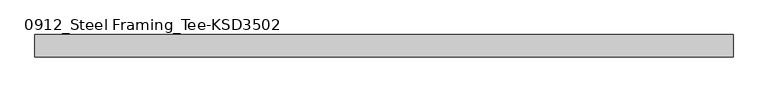
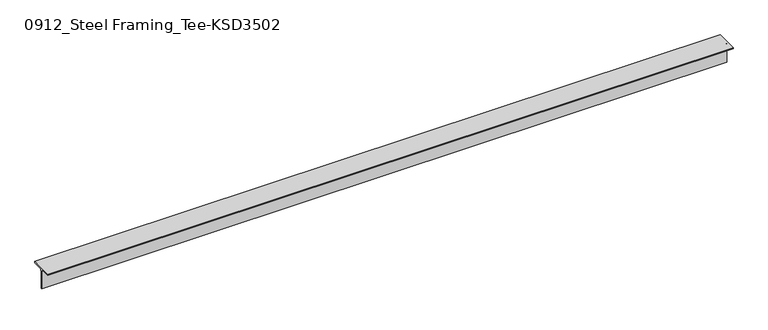
"""IFC4 building model written with IfcOpenShell, lengths in millimetres: member geometry, 0912_Steel Framing_Tee-KSD3502 : H_SB_ASB_CT-150x150x6.5x9."""

import ifcopenshell
import ifcopenshell.guid

model = None  # the IFC model being written
_history = None  # IfcOwnerHistory: only IFC2X3 demands one
_inside = {}  # id of a spatial element -> (the spatial element, [elements in it])
_under = {}  # id of a project, library or spatial element -> (it, [spatial elements below it])
_declared = {}  # id of a project -> (the project, [libraries it declares])
_typed = {}  # id of a type object -> (the type object, [elements of that type])
_made_of = {}  # id of a material, layer set ... -> (it, [elements and type objects made of it])


def new_model(schema):
    """Start an empty IFC model of exactly this schema.

    Asked for "IFC4X3", IfcOpenShell would pick the latest addendum, in which some entities
    have other attributes; the version numbers below select the first issue.
    IFC2X3 requires an IfcOwnerHistory on every rooted entity: one is made here for all.
    """
    global model, _history
    if schema == "IFC4X3":
        model = ifcopenshell.file(schema_version=(4, 3, 0, 0))
    else:
        model = ifcopenshell.file(schema=schema)
    _inside.clear()
    _under.clear()
    _declared.clear()
    _typed.clear()
    _made_of.clear()
    _history = None
    if model.schema == "IFC2X3":
        org = make("IfcOrganization", Name="unknown")
        user = make(
            "IfcPersonAndOrganization",
            ThePerson=make("IfcPerson", FamilyName="unknown"),
            TheOrganization=org,
        )
        app = make(
            "IfcApplication",
            ApplicationDeveloper=org,
            Version="unknown",
            ApplicationFullName="unknown",
            ApplicationIdentifier="unknown",
        )
        _history = make(
            "IfcOwnerHistory",
            OwningUser=user,
            OwningApplication=app,
            ChangeAction="ADDED",
            CreationDate=0,
        )
    return model


def make(cls, **values):
    """One entity of the class cls with the attributes given. An attribute that is None is left unset."""
    return model.create_entity(
        cls, **{name: value for name, value in values.items() if value is not None}
    )


def rooted(cls, **values):
    """An entity with a GlobalId (a new one), such as an element, a storey or a relation."""
    return make(cls, GlobalId=ifcopenshell.guid.new(), OwnerHistory=_history, **values)


def si_unit(unit_type, name, prefix=None):
    """IfcSIUnit, for example si_unit("LENGTHUNIT", "METRE", prefix="MILLI")."""
    return make("IfcSIUnit", UnitType=unit_type, Prefix=prefix, Name=name)


def assignment(units):
    """IfcUnitAssignment: the units of a project."""
    return None if units is None else make("IfcUnitAssignment", Units=units)


def point(xyz):
    """IfcCartesianPoint."""
    return None if xyz is None else make("IfcCartesianPoint", Coordinates=xyz)


def direction(xyz):
    """IfcDirection."""
    return None if xyz is None else make("IfcDirection", DirectionRatios=xyz)


def frame(location, z_axis=None, x_axis=None):
    """IfcAxis2Placement3D, a coordinate frame: its origin and axes. An axis left out is left unset."""
    return make(
        "IfcAxis2Placement3D",
        Location=point(location),
        Axis=direction(z_axis),
        RefDirection=direction(x_axis),
    )


def frame_2d(location, x_axis=None):
    """IfcAxis2Placement2D, a coordinate frame in the plane: its origin and x axis."""
    return make(
        "IfcAxis2Placement2D", Location=point(location), RefDirection=direction(x_axis)
    )


def origin():
    """The frame at (0, 0, 0) with its axes left unset."""
    return frame((0.0, 0.0, 0.0))


def place(relative_to, where):
    """IfcLocalPlacement: puts the frame where relative to a parent placement (None: the world)."""
    return make(
        "IfcLocalPlacement", PlacementRelTo=relative_to, RelativePlacement=where
    )


def context(
    kind, dimensions, precision=None, world=None, true_north=None, identifier=None
):
    """IfcGeometricRepresentationContext, for example the 3D "Model" context."""
    return make(
        "IfcGeometricRepresentationContext",
        ContextIdentifier=identifier,
        ContextType=kind,
        CoordinateSpaceDimension=dimensions,
        Precision=precision,
        WorldCoordinateSystem=world,
        TrueNorth=true_north,
    )


def project(units=None, contexts=None):
    """IfcProject with its units and contexts."""
    return rooted(
        "IfcProject",
        Name="project",
        RepresentationContexts=contexts,
        UnitsInContext=assignment(units),
    )


def spatial(cls, under=None, at=None, **own):
    """A site, building, storey or space (cls), placed at a placement, below another one or the project."""
    s = rooted(cls, ObjectPlacement=at, **own)
    if under is not None:
        _under.setdefault(under.id(), (under, []))[1].append(s)
    return s


def polyline(points):
    """IfcPolyline through the points."""
    return make("IfcPolyline", Points=[point(p) for p in points])


def circle_curve(where, radius):
    """IfcCircle in the frame where."""
    return make("IfcCircle", Position=where, Radius=radius)


def trimmed(basis, trim1, trim2, sense, master):
    """IfcTrimmedCurve: the piece of a basis curve between two trims."""
    return make(
        "IfcTrimmedCurve",
        BasisCurve=basis,
        Trim1=trim1,
        Trim2=trim2,
        SenseAgreement=sense,
        MasterRepresentation=master,
    )


def segment(curve, same_sense, transition):
    """IfcCompositeCurveSegment."""
    return make(
        "IfcCompositeCurveSegment",
        Transition=transition,
        SameSense=same_sense,
        ParentCurve=curve,
    )


def composite_curve(segments, self_intersect=None):
    """IfcCompositeCurve: segments joined end to end."""
    return make("IfcCompositeCurve", Segments=segments, SelfIntersect=self_intersect)


def outline(outer, holes=None, kind="AREA"):
    """IfcArbitraryClosedProfileDef: a profile drawn as a closed curve; with holes, ...WithVoids."""
    if holes is None:
        return make("IfcArbitraryClosedProfileDef", ProfileType=kind, OuterCurve=outer)
    return make(
        "IfcArbitraryProfileDefWithVoids",
        ProfileType=kind,
        OuterCurve=outer,
        InnerCurves=holes,
    )


def extrude(swept, where, along, depth):
    """IfcExtrudedAreaSolid: the profile swept, set in the frame where, extruded along a direction by depth."""
    return make(
        "IfcExtrudedAreaSolid",
        SweptArea=swept,
        Position=where,
        ExtrudedDirection=direction(along),
        Depth=depth,
    )


def shape(context_of_items, identifier, shape_type, items):
    """IfcShapeRepresentation: the items that make up one representation, for example the "Body"."""
    return make(
        "IfcShapeRepresentation",
        ContextOfItems=context_of_items,
        RepresentationIdentifier=identifier,
        RepresentationType=shape_type,
        Items=items,
    )


def source(mapping_origin, context_of_items, identifier, shape_type, items):
    """IfcRepresentationMap: a shape defined once, which mapped items show again and again."""
    return make(
        "IfcRepresentationMap",
        MappingOrigin=mapping_origin,
        MappedRepresentation=shape(context_of_items, identifier, shape_type, items),
    )


def transform(
    local_origin,
    x_axis=None,
    y_axis=None,
    z_axis=None,
    scale=None,
    scale2=None,
    scale3=None,
    uniform=True,
):
    """IfcCartesianTransformationOperator3D, or its non-uniform kind. x_axis, y_axis, z_axis: its Axis1, 2, 3."""
    if uniform:
        return make(
            "IfcCartesianTransformationOperator3D",
            Axis1=direction(x_axis),
            Axis2=direction(y_axis),
            LocalOrigin=point(local_origin),
            Scale=scale,
            Axis3=direction(z_axis),
        )
    return make(
        "IfcCartesianTransformationOperator3DnonUniform",
        Axis1=direction(x_axis),
        Axis2=direction(y_axis),
        LocalOrigin=point(local_origin),
        Scale=scale,
        Axis3=direction(z_axis),
        Scale2=scale2,
        Scale3=scale3,
    )


def mapped(mapping_source, mapping_target):
    """IfcMappedItem: shows the shape of a source again, moved by a transform."""
    return make(
        "IfcMappedItem", MappingSource=mapping_source, MappingTarget=mapping_target
    )


def made_of(thing, what):
    """Note that an element or type object is made of a material, layer set ...; save() writes the relation."""
    if what is not None:
        _made_of.setdefault(what.id(), (what, []))[1].append(thing)
    return thing


def element(
    cls,
    number,
    at=None,
    inside=None,
    cuts=None,
    type_object=None,
    material=None,
    context=None,
    identifier="Body",
    shape_type=None,
    held_by="IfcProductDefinitionShape",
    body=None,
    shapes=None,
    **own,
):
    """One element of the class cls, such as IfcWall. Its Tag is "e" and its number.

    at: its placement. inside: the storey or other place that contains it. cuts: it is an
    opening in that element (IfcRelVoidsElement). A single representation is given by context,
    identifier, shape_type and body (its items); several are given by shapes. held_by: the class
    of the entity that holds the representations. save() writes the other relations.
    """
    e = rooted(cls, Tag="e%d" % number, ObjectPlacement=at, **own)
    if body is not None:
        shapes = [shape(context, identifier, shape_type, body)]
    if shapes is not None:
        e.Representation = make(held_by, Representations=shapes)
    if inside is not None:
        _inside.setdefault(inside.id(), (inside, []))[1].append(e)
    if cuts is not None:
        rooted(
            "IfcRelVoidsElement", RelatingBuildingElement=cuts, RelatedOpeningElement=e
        )
    if type_object is not None:
        _typed.setdefault(type_object.id(), (type_object, []))[1].append(e)
    return made_of(e, material)


def aggregate(whole, parts):
    """IfcRelAggregates: a whole, such as a stair, and the parts it consists of."""
    return rooted("IfcRelAggregates", RelatingObject=whole, RelatedObjects=parts)


def save(model, path):
    """Write the relations noted so far, then the file.

    IfcRelAggregates (storeys below a building ...), IfcRelContainedInSpatialStructure (elements
    in a storey), IfcRelDefinesByType, IfcRelAssociatesMaterial and IfcRelDeclares: one each for
    every whole, place, type object, material and project.
    """
    for whole, parts in _under.values():
        aggregate(whole, parts)
    for where, things in _inside.values():
        rooted(
            "IfcRelContainedInSpatialStructure",
            RelatedElements=things,
            RelatingStructure=where,
        )
    for kind, things in _typed.values():
        rooted("IfcRelDefinesByType", RelatedObjects=things, RelatingType=kind)
    for what, things in _made_of.values():
        rooted("IfcRelAssociatesMaterial", RelatedObjects=things, RelatingMaterial=what)
    for by, libraries in _declared.values():
        rooted("IfcRelDeclares", RelatingContext=by, RelatedDefinitions=libraries)
    model.write(path)


def member_0912_steel_framing_tee_ksd3502_358c1067(model_context):
    return source(origin(), model_context, "Body", "SweptSolid", [
        extrude(outline(composite_curve([segment(polyline([(-75.0, 75.0), (75.0, 75.0), (75.0, 66.0), (16.25, 66.0)]), True, "CONTINUOUS"), segment(trimmed(circle_curve(frame_2d((16.25, 53.0)), 13.0), [point((16.25, 66.0))], [point((3.25, 53.0))], True, "CARTESIAN"), True, "CONTINUOUS"), segment(polyline([(3.25, 53.0), (3.25, -75.0), (-3.25, -75.0), (-3.25, 53.0)]), True, "CONTINUOUS"), segment(trimmed(circle_curve(frame_2d((-16.25, 53.0)), 13.0), [point((-3.25, 53.0))], [point((-16.25, 66.0))], True, "CARTESIAN"), True, "CONTINUOUS"), segment(polyline([(-16.25, 66.0), (-75.0, 66.0), (-75.0, 75.0)]), True, "CONTINUOUS")], self_intersect=False)), frame((-2342.2, 0.0, 0.0), z_axis=(1.0, 0.0, 0.0), x_axis=(0.0, 1.0, 0.0)), (0.0, 0.0, 1.0), 4645.3),
    ])


if __name__ == "__main__":
    model = new_model("IFC4")
    model_context = context("Model", 3, world=origin())
    ifc_project = project(units=[si_unit("LENGTHUNIT", "METRE", prefix="MILLI")], contexts=[model_context])
    site = spatial("IfcSite", under=ifc_project)
    building = spatial("IfcBuilding", under=site)
    placement = place(None, origin())
    member_0912_steel_framing_tee_ksd3502_shape = member_0912_steel_framing_tee_ksd3502_358c1067(model_context)
    element("IfcMember", 1, ObjectType="0912_Steel Framing_Tee-KSD3502 : H_SB_ASB_CT-150x150x6.5x9", at=placement, inside=building, context=model_context, shape_type="MappedRepresentation", body=[
        mapped(member_0912_steel_framing_tee_ksd3502_shape, transform((0.0, 0.0, 0.0), x_axis=(1.0, 0.0, 0.0), y_axis=(0.0, 1.0, 0.0), z_axis=(0.0, 0.0, 1.0))),
    ])
    save(model, "model.ifc")

# Revit data of these elements
# Type "0912_Steel Framing_Tee-KSD3502 : H_SB_ASB_CT-150x150x6.5x9"
#   H_WM Code_1 = "S01AA003-00001 | Main Steel Structure Fabrication Work | Shelter/Building | Light Steel - Standard (30KG/M>Weight) | Material: (   )"
#   H_WM Code_2 = "S03AA029-00001 | Main Steel Structure Erection Work | Shelter/Building | Light Steel (30KG/M>Weight) | Material: (   )"
#   H_WM Code_3 = "S01AA010-00001 | Main Steel Structure Fabrication Work | Shelter/Building | Steel Painting/Coating | for Non-Fireproofed Steel Surface, Surface Preparation, Primer, Second & Final Coat | Material: (   )"
#   H_Q'ty Cal Type Tag = "SB-Q2"
#   Width = 15.0 cm
#   Web Thickness = 0.65 cm
#   Web Fillet = 1.3 cm
#   Section Area = 23.39 cm²
#   Perimeter = 0.60 m²/m
#   Nominal Weight = 18.40 kgf/m
#   Height = 15.0 cm
#   Flange Thickness = 0.9 cm
#   Centroid Vertical = 7.5 cm
#   Centroid Horizontal = 7.5 cm
#   Length [instance default] = 1.5000 m
#   Structural Material [instance default] = Steel, 45-345
#   Warping Constant = (empty or 0)
#   Torsional Moment of Inertia = 0
#   Section Name Key = ""
#   Plastic Modulus weak axis = 0
#   Plastic Modulus strong axis = 0
#   Moment of Inertia weak axis = 0
#   Moment of Inertia strong axis = 0
#   Elastic Modulus weak axis = 0
#   Elastic Modulus strong axis = 0
#   Bolt Spacing = 0
#   Assembly Code = ""
# Element 1 (IfcMember, "0912_Steel Framing_Tee-KSD3502 : H_SB_ASB_CT-150x150x6.5x9")
#   Structural Material = none
# Materials
#   "Steel, 45-345": class "Metal", colour RGB 189 187 185, transparency 0, Description = "Steel 345 MPa", Cost = 0
